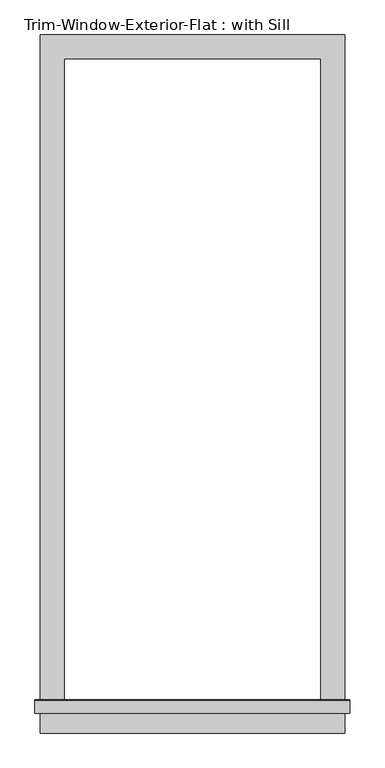
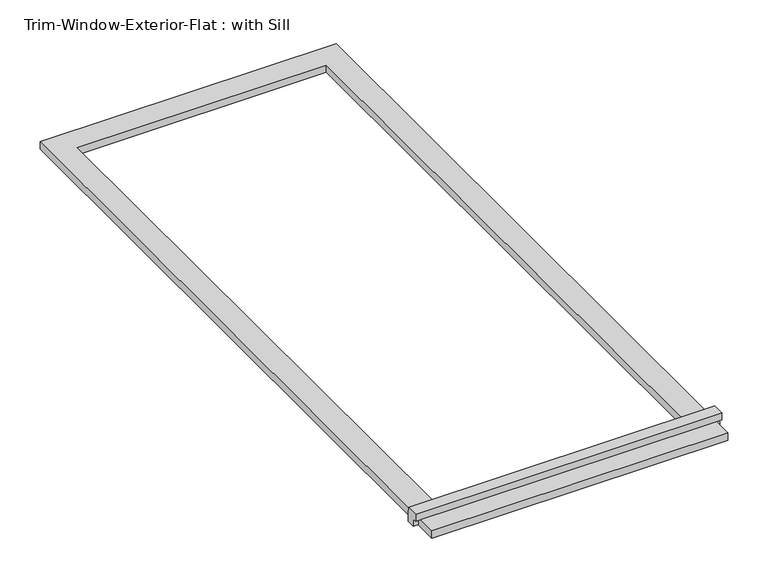
"""IFC4 building model written with IfcOpenShell, lengths in millimetres: proxy geometry, Trim-Window-Exterior-Flat : with Sill."""

import ifcopenshell
import ifcopenshell.guid

model = None  # the IFC model being written
_history = None  # IfcOwnerHistory: only IFC2X3 demands one
_inside = {}  # id of a spatial element -> (the spatial element, [elements in it])
_under = {}  # id of a project, library or spatial element -> (it, [spatial elements below it])
_declared = {}  # id of a project -> (the project, [libraries it declares])
_typed = {}  # id of a type object -> (the type object, [elements of that type])
_made_of = {}  # id of a material, layer set ... -> (it, [elements and type objects made of it])


def new_model(schema):
    """Start an empty IFC model of exactly this schema.

    Asked for "IFC4X3", IfcOpenShell would pick the latest addendum, in which some entities
    have other attributes; the version numbers below select the first issue.
    IFC2X3 requires an IfcOwnerHistory on every rooted entity: one is made here for all.
    """
    global model, _history
    if schema == "IFC4X3":
        model = ifcopenshell.file(schema_version=(4, 3, 0, 0))
    else:
        model = ifcopenshell.file(schema=schema)
    _inside.clear()
    _under.clear()
    _declared.clear()
    _typed.clear()
    _made_of.clear()
    _history = None
    if model.schema == "IFC2X3":
        org = make("IfcOrganization", Name="unknown")
        user = make(
            "IfcPersonAndOrganization",
            ThePerson=make("IfcPerson", FamilyName="unknown"),
            TheOrganization=org,
        )
        app = make(
            "IfcApplication",
            ApplicationDeveloper=org,
            Version="unknown",
            ApplicationFullName="unknown",
            ApplicationIdentifier="unknown",
        )
        _history = make(
            "IfcOwnerHistory",
            OwningUser=user,
            OwningApplication=app,
            ChangeAction="ADDED",
            CreationDate=0,
        )
    return model


def make(cls, **values):
    """One entity of the class cls with the attributes given. An attribute that is None is left unset."""
    return model.create_entity(
        cls, **{name: value for name, value in values.items() if value is not None}
    )


def rooted(cls, **values):
    """An entity with a GlobalId (a new one), such as an element, a storey or a relation."""
    return make(cls, GlobalId=ifcopenshell.guid.new(), OwnerHistory=_history, **values)


def si_unit(unit_type, name, prefix=None):
    """IfcSIUnit, for example si_unit("LENGTHUNIT", "METRE", prefix="MILLI")."""
    return make("IfcSIUnit", UnitType=unit_type, Prefix=prefix, Name=name)


def assignment(units):
    """IfcUnitAssignment: the units of a project."""
    return None if units is None else make("IfcUnitAssignment", Units=units)


def point(xyz):
    """IfcCartesianPoint."""
    return None if xyz is None else make("IfcCartesianPoint", Coordinates=xyz)


def direction(xyz):
    """IfcDirection."""
    return None if xyz is None else make("IfcDirection", DirectionRatios=xyz)


def frame(location, z_axis=None, x_axis=None):
    """IfcAxis2Placement3D, a coordinate frame: its origin and axes. An axis left out is left unset."""
    return make(
        "IfcAxis2Placement3D",
        Location=point(location),
        Axis=direction(z_axis),
        RefDirection=direction(x_axis),
    )


def origin():
    """The frame at (0, 0, 0) with its axes left unset."""
    return frame((0.0, 0.0, 0.0))


def origin_with_axes():
    """The frame at (0, 0, 0) with the z axis (0, 0, 1) and the x axis (1, 0, 0) written out."""
    return frame((0.0, 0.0, 0.0), z_axis=(0.0, 0.0, 1.0), x_axis=(1.0, 0.0, 0.0))


def place(relative_to, where):
    """IfcLocalPlacement: puts the frame where relative to a parent placement (None: the world)."""
    return make(
        "IfcLocalPlacement", PlacementRelTo=relative_to, RelativePlacement=where
    )


def context(
    kind, dimensions, precision=None, world=None, true_north=None, identifier=None
):
    """IfcGeometricRepresentationContext, for example the 3D "Model" context."""
    return make(
        "IfcGeometricRepresentationContext",
        ContextIdentifier=identifier,
        ContextType=kind,
        CoordinateSpaceDimension=dimensions,
        Precision=precision,
        WorldCoordinateSystem=world,
        TrueNorth=true_north,
    )


def project(units=None, contexts=None):
    """IfcProject with its units and contexts."""
    return rooted(
        "IfcProject",
        Name="project",
        RepresentationContexts=contexts,
        UnitsInContext=assignment(units),
    )


def spatial(cls, under=None, at=None, **own):
    """A site, building, storey or space (cls), placed at a placement, below another one or the project."""
    s = rooted(cls, ObjectPlacement=at, **own)
    if under is not None:
        _under.setdefault(under.id(), (under, []))[1].append(s)
    return s


def polyline(points):
    """IfcPolyline through the points."""
    return make("IfcPolyline", Points=[point(p) for p in points])


def outline(outer, holes=None, kind="AREA"):
    """IfcArbitraryClosedProfileDef: a profile drawn as a closed curve; with holes, ...WithVoids."""
    if holes is None:
        return make("IfcArbitraryClosedProfileDef", ProfileType=kind, OuterCurve=outer)
    return make(
        "IfcArbitraryProfileDefWithVoids",
        ProfileType=kind,
        OuterCurve=outer,
        InnerCurves=holes,
    )


def extrude(swept, where, along, depth):
    """IfcExtrudedAreaSolid: the profile swept, set in the frame where, extruded along a direction by depth."""
    return make(
        "IfcExtrudedAreaSolid",
        SweptArea=swept,
        Position=where,
        ExtrudedDirection=direction(along),
        Depth=depth,
    )


def shape(context_of_items, identifier, shape_type, items):
    """IfcShapeRepresentation: the items that make up one representation, for example the "Body"."""
    return make(
        "IfcShapeRepresentation",
        ContextOfItems=context_of_items,
        RepresentationIdentifier=identifier,
        RepresentationType=shape_type,
        Items=items,
    )


def source(mapping_origin, context_of_items, identifier, shape_type, items):
    """IfcRepresentationMap: a shape defined once, which mapped items show again and again."""
    return make(
        "IfcRepresentationMap",
        MappingOrigin=mapping_origin,
        MappedRepresentation=shape(context_of_items, identifier, shape_type, items),
    )


def transform(
    local_origin,
    x_axis=None,
    y_axis=None,
    z_axis=None,
    scale=None,
    scale2=None,
    scale3=None,
    uniform=True,
):
    """IfcCartesianTransformationOperator3D, or its non-uniform kind. x_axis, y_axis, z_axis: its Axis1, 2, 3."""
    if uniform:
        return make(
            "IfcCartesianTransformationOperator3D",
            Axis1=direction(x_axis),
            Axis2=direction(y_axis),
            LocalOrigin=point(local_origin),
            Scale=scale,
            Axis3=direction(z_axis),
        )
    return make(
        "IfcCartesianTransformationOperator3DnonUniform",
        Axis1=direction(x_axis),
        Axis2=direction(y_axis),
        LocalOrigin=point(local_origin),
        Scale=scale,
        Axis3=direction(z_axis),
        Scale2=scale2,
        Scale3=scale3,
    )


def mapped(mapping_source, mapping_target):
    """IfcMappedItem: shows the shape of a source again, moved by a transform."""
    return make(
        "IfcMappedItem", MappingSource=mapping_source, MappingTarget=mapping_target
    )


def made_of(thing, what):
    """Note that an element or type object is made of a material, layer set ...; save() writes the relation."""
    if what is not None:
        _made_of.setdefault(what.id(), (what, []))[1].append(thing)
    return thing


def element(
    cls,
    number,
    at=None,
    inside=None,
    cuts=None,
    type_object=None,
    material=None,
    context=None,
    identifier="Body",
    shape_type=None,
    held_by="IfcProductDefinitionShape",
    body=None,
    shapes=None,
    **own,
):
    """One element of the class cls, such as IfcWall. Its Tag is "e" and its number.

    at: its placement. inside: the storey or other place that contains it. cuts: it is an
    opening in that element (IfcRelVoidsElement). A single representation is given by context,
    identifier, shape_type and body (its items); several are given by shapes. held_by: the class
    of the entity that holds the representations. save() writes the other relations.
    """
    e = rooted(cls, Tag="e%d" % number, ObjectPlacement=at, **own)
    if body is not None:
        shapes = [shape(context, identifier, shape_type, body)]
    if shapes is not None:
        e.Representation = make(held_by, Representations=shapes)
    if inside is not None:
        _inside.setdefault(inside.id(), (inside, []))[1].append(e)
    if cuts is not None:
        rooted(
            "IfcRelVoidsElement", RelatingBuildingElement=cuts, RelatedOpeningElement=e
        )
    if type_object is not None:
        _typed.setdefault(type_object.id(), (type_object, []))[1].append(e)
    return made_of(e, material)


def aggregate(whole, parts):
    """IfcRelAggregates: a whole, such as a stair, and the parts it consists of."""
    return rooted("IfcRelAggregates", RelatingObject=whole, RelatedObjects=parts)


def save(model, path):
    """Write the relations noted so far, then the file.

    IfcRelAggregates (storeys below a building ...), IfcRelContainedInSpatialStructure (elements
    in a storey), IfcRelDefinesByType, IfcRelAssociatesMaterial and IfcRelDeclares: one each for
    every whole, place, type object, material and project.
    """
    for whole, parts in _under.values():
        aggregate(whole, parts)
    for where, things in _inside.values():
        rooted(
            "IfcRelContainedInSpatialStructure",
            RelatedElements=things,
            RelatingStructure=where,
        )
    for kind, things in _typed.values():
        rooted("IfcRelDefinesByType", RelatedObjects=things, RelatingType=kind)
    for what, things in _made_of.values():
        rooted("IfcRelAssociatesMaterial", RelatedObjects=things, RelatingMaterial=what)
    for by, libraries in _declared.values():
        rooted("IfcRelDeclares", RelatingContext=by, RelatedDefinitions=libraries)
    model.write(path)


def trim_window_exterior_flat_with_sill_4912eb0d(model_context):
    return source(origin(), model_context, "Body", "SweptSolid", [
        extrude(outline(polyline([(361.95, -1546.1823709), (361.95, -1603.3323709), (-361.95, -1603.3323709), (-361.95, -1546.1823709), (361.95, -1546.1823709)])), origin_with_axes(), (0.0, 0.0, 1.0), 19.05),
        extrude(outline(polyline([(-1555.75, 38.1), (-1526.4580645, 38.1), (-1524.0, 19.05), (-1524.0, 0.0), (-1546.1823709, 0.0), (-1546.1823709, 19.05), (-1555.75, 19.05), (-1555.75, 38.1)])), frame((-374.65, 0.0, 0.0), z_axis=(1.0, 0.0, 0.0), x_axis=(0.0, 1.0, 0.0)), (0.0, 0.0, 1.0), 749.3),
        extrude(outline(polyline([(-361.95, 57.15), (361.95, 57.15), (361.95, -1524.0), (304.8, -1524.0), (304.8, 0.0), (-304.8, 0.0), (-304.8, -1524.0), (-361.95, -1524.0), (-361.95, 57.15)])), origin_with_axes(), (0.0, 0.0, 1.0), 19.05),
    ])


if __name__ == "__main__":
    model = new_model("IFC4")
    model_context = context("Model", 3, world=origin())
    ifc_project = project(units=[si_unit("LENGTHUNIT", "METRE", prefix="MILLI")], contexts=[model_context])
    site = spatial("IfcSite", under=ifc_project)
    building = spatial("IfcBuilding", under=site)
    placement = place(None, origin())
    trim_window_exterior_flat_with_sill_shape = trim_window_exterior_flat_with_sill_4912eb0d(model_context)
    element("IfcBuildingElementProxy", 1, Name="Trim-Window-Exterior-Flat : with Sill", ObjectType="Trim-Window-Exterior-Flat : with Sill", at=placement, inside=building, context=model_context, shape_type="MappedRepresentation", body=[
        mapped(trim_window_exterior_flat_with_sill_shape, transform((0.0, 0.0, 0.0), x_axis=(1.0, 0.0, 0.0), y_axis=(0.0, 1.0, 0.0), z_axis=(0.0, 0.0, 1.0))),
    ])
    save(model, "model.ifc")

# Revit data of these elements
# Type "Trim-Window-Exterior-Flat : with Sill"
#   Trim Width = 0' - 2 1/4"
#   Trim Thickness_Picture Frame = 0' - 1 1/4"
#   Trim Thickness_with Sill = 0' - 0 3/4"
#   Sill Thickness = 0' - 1 1/4"
#   Opening Width [instance default] = 2' - 0"
#   Opening Height [instance default] = 3' - 0"
#   Default Elevation = 4' - 0"
#   Sill = yes
#   Picture Frame = no
#   Trim Material [instance default] = none
# Element 1 (IfcBuildingElementProxy, "Trim-Window-Exterior-Flat : with Sill")
#   Opening Height = 5' - 0"
#   Trim Material = Clad - White
#   Materials on its faces: "Clad - White"
# Materials
#   "Clad - White": class "Wood", colour RGB 242 242 238, transparency 0, Cost = 0
